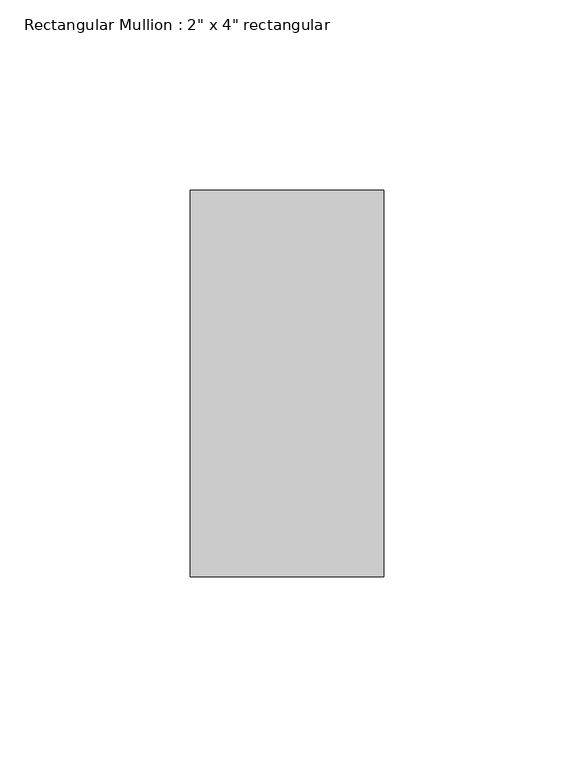
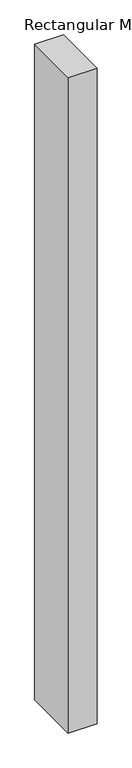
"""IFC4 building model written with IfcOpenShell, lengths in millimetres: member geometry."""

from ifc_helpers import new_model, si_unit, frame, origin, place, context, project, spatial, polyline, outline, extrude, source, transform, mapped, element, save


def member_0adc4f37(model_context):
    return source(origin(), model_context, "Body", "SweptSolid", [
        extrude(outline(polyline([(0.0, 50.8), (0.0, -50.8), (-50.8, -50.8), (-50.8, 50.8), (0.0, 50.8)])), frame((0.0, 0.0, -1219.2), z_axis=(0.0, 0.0, 1.0), x_axis=(1.0, 0.0, 0.0)), (0.0, 0.0, 1.0), 1219.2),
    ])


if __name__ == "__main__":
    model = new_model("IFC4")
    model_context = context("Model", 3, world=origin())
    ifc_project = project(units=[si_unit("LENGTHUNIT", "METRE", prefix="MILLI")], contexts=[model_context])
    site = spatial("IfcSite", under=ifc_project)
    building = spatial("IfcBuilding", under=site)
    placement = place(None, origin())
    member_shape = member_0adc4f37(model_context)
    element("IfcMember", 1, ObjectType="Rectangular Mullion : 2\" x 4\" rectangular", at=placement, inside=building, context=model_context, shape_type="MappedRepresentation", body=[
        mapped(member_shape, transform((0.0, 0.0, 0.0), x_axis=(1.0, 0.0, 0.0), y_axis=(0.0, 1.0, 0.0), z_axis=(0.0, 0.0, 1.0))),
    ])
    save(model, "model.ifc")

# Revit data of these elements
# Type "Rectangular Mullion : 2\" x 4\" rectangular"
#   built-in parameter 1007304 = 0.333333 (stored number, unit not read)
#   built-in parameter 1007301 = 0.0833333 (stored number, unit not read)
#   built-in parameter 1007300 = 0.0833333 (stored number, unit not read)
